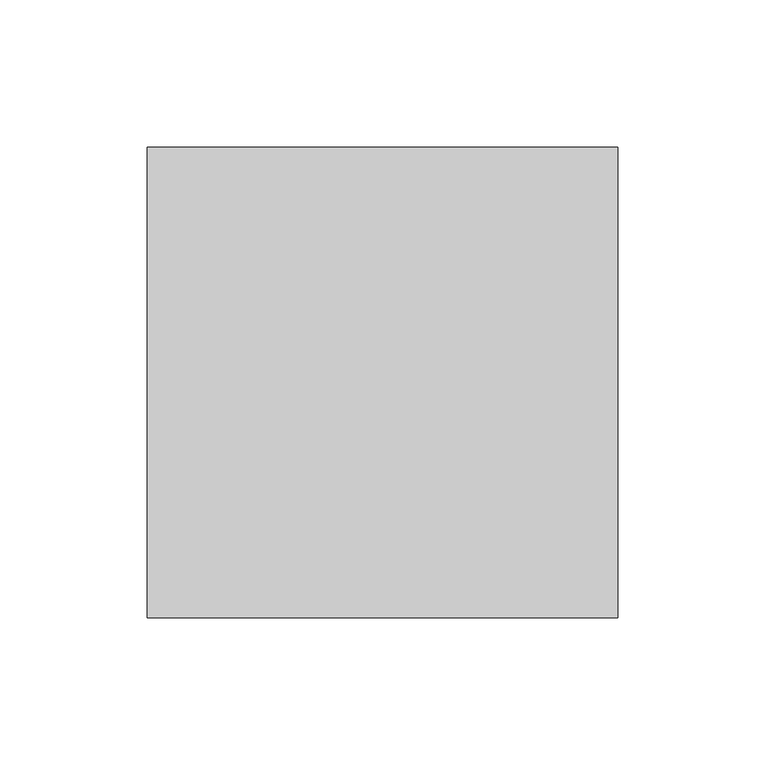
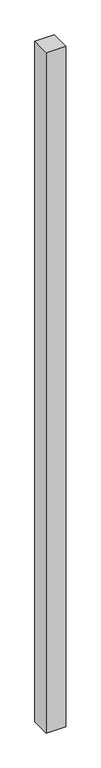
"""IFC4 building model written with IfcOpenShell, lengths in millimetres: column geometry, 0_3d."""

from ifc_helpers import new_model, si_unit, origin, origin_with_axes, place, context, project, spatial, polyline, outline, extrude, source, transform, mapped, element, save


def column_19bb80a0(model_context):
    return source(origin(), model_context, "Body", "SweptSolid", [
        extrude(outline(polyline([(160.0, 160.0), (160.0, 0.0), (0.0, 0.0), (0.0, 160.0), (160.0, 160.0)])), origin_with_axes(), (0.0, 0.0, 1.0), 5880.0),
    ])


if __name__ == "__main__":
    model = new_model("IFC4")
    model_context = context("Model", 3, world=origin())
    ifc_project = project(units=[si_unit("LENGTHUNIT", "METRE", prefix="MILLI")], contexts=[model_context])
    site = spatial("IfcSite", under=ifc_project)
    building = spatial("IfcBuilding", under=site)
    placement = place(None, origin())
    column_shape = column_19bb80a0(model_context)
    element("IfcColumn", 1, ObjectType="0_3d", at=placement, inside=building, context=model_context, shape_type="MappedRepresentation", body=[
        mapped(column_shape, transform((0.0, 0.0, 0.0), x_axis=(1.0, 0.0, 0.0), y_axis=(0.0, 1.0, 0.0), z_axis=(0.0, 0.0, 1.0))),
    ])
    save(model, "model.ifc")

# Revit data of these elements
# Element 1 (IfcColumn, "0_3d")
#   Materials on its faces: "material wardrobe b 1"
# Materials
#   "material wardrobe b 1": class "Unassigned", colour RGB 128 128 128, transparency 0
